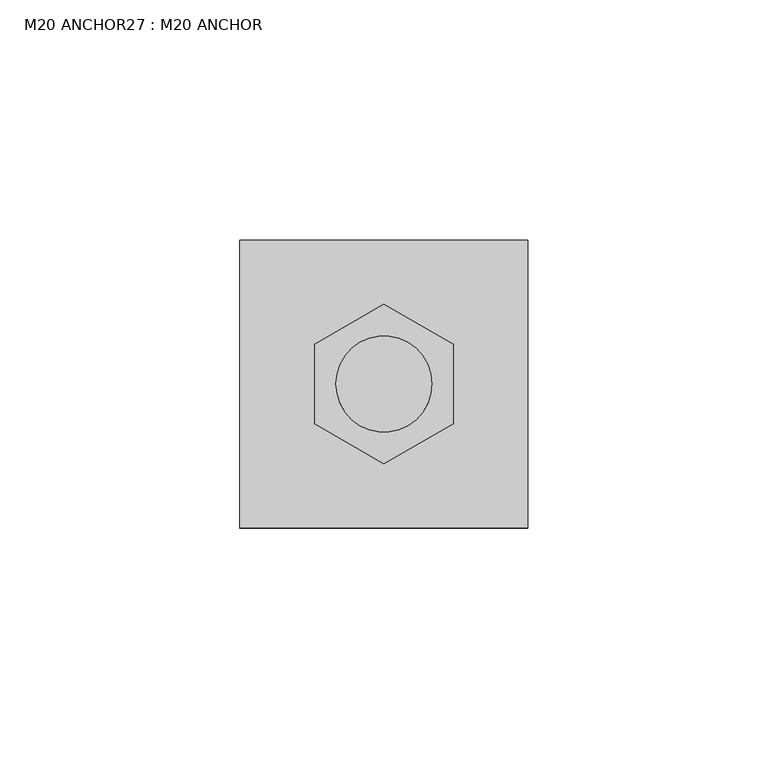
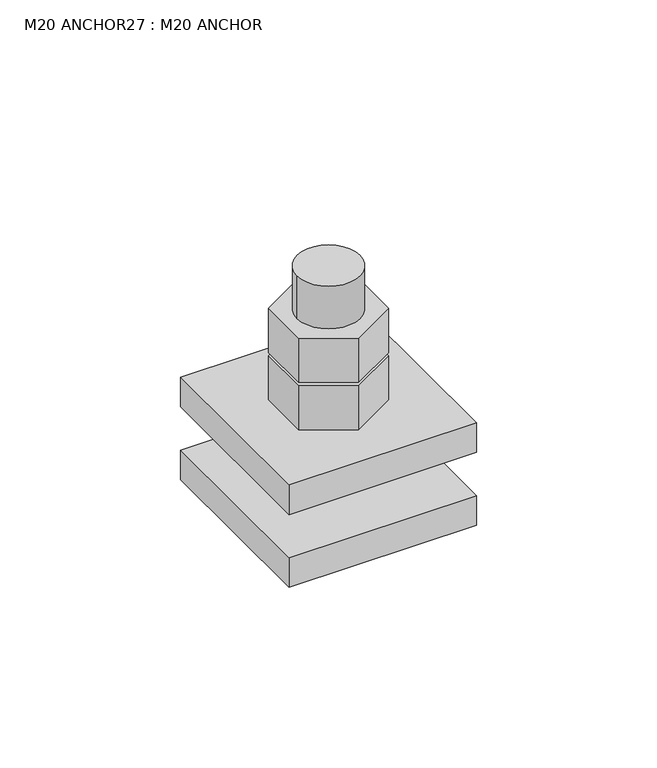
"""IFC4 building model written with IfcOpenShell, lengths in millimetres: fastener geometry, M20 ANCHOR27 : M20 ANCHOR."""

from ifc_helpers import new_model, si_unit, point, frame, frame_2d, origin, place, context, project, spatial, polyline, circle_curve, trimmed, segment, composite_curve, outline, extrude, source, transform, mapped, element, save


def m20_anchor27_m20_anchor_028f3715(model_context):
    return source(origin(), model_context, "Body", "SweptSolid", [
        extrude(outline(polyline([(-30672.4939916, -7533.2988347), (-30686.9021106, -7541.6173661), (-30701.3102297, -7533.2988347), (-30701.3102297, -7516.6617719), (-30686.9021106, -7508.3432405), (-30672.4939916, -7516.6617719), (-30672.4939916, -7533.2988347)]), holes=[composite_curve([segment(trimmed(circle_curve(frame_2d((-30686.9021106, -7524.9803033)), 10.0), [point((-30696.9021106, -7524.9803033))], [point((-30676.9021106, -7524.9803033))], True, "CARTESIAN"), True, "CONTINUOUS"), segment(trimmed(circle_curve(frame_2d((-30686.9021106, -7524.9803033)), 10.0), [point((-30676.9021106, -7524.9803033))], [point((-30696.9021106, -7524.9803033))], True, "CARTESIAN"), True, "CONTINUOUS")], self_intersect=False)]), frame((0.0, 0.0, 240.605), z_axis=(0.0, 0.0, 1.0), x_axis=(1.0, 0.0, 0.0)), (0.0, 0.0, 1.0), 15.0),
        extrude(outline(polyline([(-30672.4939916, -7533.2988347), (-30686.9021106, -7541.6173661), (-30701.3102297, -7533.2988347), (-30701.3102297, -7516.6617719), (-30686.9021106, -7508.3432405), (-30672.4939916, -7516.6617719), (-30672.4939916, -7533.2988347)]), holes=[composite_curve([segment(trimmed(circle_curve(frame_2d((-30686.9021106, -7524.9803033)), 10.0), [point((-30696.9021106, -7524.9803033))], [point((-30676.9021106, -7524.9803033))], True, "CARTESIAN"), True, "CONTINUOUS"), segment(trimmed(circle_curve(frame_2d((-30686.9021106, -7524.9803033)), 10.0), [point((-30676.9021106, -7524.9803033))], [point((-30696.9021106, -7524.9803033))], True, "CARTESIAN"), True, "CONTINUOUS")], self_intersect=False)]), frame((0.0, 0.0, 224.605), z_axis=(0.0, 0.0, 1.0), x_axis=(1.0, 0.0, 0.0)), (0.0, 0.0, 1.0), 15.0),
        extrude(outline(composite_curve([segment(trimmed(circle_curve(frame_2d((-30686.9021106, -7524.9803033)), 10.0), [point((-30696.9021106, -7524.9803033))], [point((-30676.9021106, -7524.9803033))], False, "CARTESIAN"), True, "CONTINUOUS"), segment(trimmed(circle_curve(frame_2d((-30686.9021106, -7524.9803033)), 10.0), [point((-30676.9021106, -7524.9803033))], [point((-30696.9021106, -7524.9803033))], False, "CARTESIAN"), True, "CONTINUOUS")], self_intersect=False)), frame((0.0, 0.0, 190.0), z_axis=(0.0, 0.0, 1.0), x_axis=(1.0, 0.0, 0.0)), (0.0, 0.0, 1.0), 80.0),
        extrude(outline(polyline([(-30656.9021106, -7554.9803033), (-30716.9021106, -7554.9803033), (-30716.9021106, -7494.9803033), (-30656.9021106, -7494.9803033), (-30656.9021106, -7554.9803033)]), holes=[composite_curve([segment(trimmed(circle_curve(frame_2d((-30686.9021106, -7524.9803033)), 11.0), [point((-30697.9021106, -7524.9803033))], [point((-30675.9021106, -7524.9803033))], True, "CARTESIAN"), True, "CONTINUOUS"), segment(trimmed(circle_curve(frame_2d((-30686.9021106, -7524.9803033)), 11.0), [point((-30675.9021106, -7524.9803033))], [point((-30697.9021106, -7524.9803033))], True, "CARTESIAN"), True, "CONTINUOUS")], self_intersect=False)]), frame((0.0, 0.0, 190.0), z_axis=(0.0, 0.0, 1.0), x_axis=(1.0, 0.0, 0.0)), (0.0, 0.0, 1.0), 10.0),
        extrude(outline(polyline([(-30656.9021106, -7554.9803033), (-30716.9021106, -7554.9803033), (-30716.9021106, -7494.9803033), (-30656.9021106, -7494.9803033), (-30656.9021106, -7554.9803033)]), holes=[composite_curve([segment(trimmed(circle_curve(frame_2d((-30686.9021106, -7524.9803033)), 11.0), [point((-30697.9021106, -7524.9803033))], [point((-30675.9021106, -7524.9803033))], True, "CARTESIAN"), True, "CONTINUOUS"), segment(trimmed(circle_curve(frame_2d((-30686.9021106, -7524.9803033)), 11.0), [point((-30675.9021106, -7524.9803033))], [point((-30697.9021106, -7524.9803033))], True, "CARTESIAN"), True, "CONTINUOUS")], self_intersect=False)]), frame((0.0, 0.0, 214.605), z_axis=(0.0, 0.0, 1.0), x_axis=(1.0, 0.0, 0.0)), (0.0, 0.0, 1.0), 10.0),
    ])


if __name__ == "__main__":
    model = new_model("IFC4")
    model_context = context("Model", 3, world=origin())
    ifc_project = project(units=[si_unit("LENGTHUNIT", "METRE", prefix="MILLI")], contexts=[model_context])
    site = spatial("IfcSite", under=ifc_project)
    building = spatial("IfcBuilding", under=site)
    placement = place(None, origin())
    m20_anchor27_m20_anchor_shape = m20_anchor27_m20_anchor_028f3715(model_context)
    element("IfcFastener", 1, ObjectType="M20 ANCHOR27 : M20 ANCHOR", at=placement, inside=building, context=model_context, shape_type="MappedRepresentation", body=[
        mapped(m20_anchor27_m20_anchor_shape, transform((0.0, 0.0, 0.0), x_axis=(1.0, 0.0, 0.0), y_axis=(0.0, 1.0, 0.0), z_axis=(0.0, 0.0, 1.0))),
    ])
    save(model, "model.ifc")
